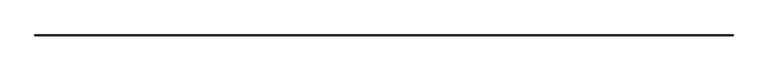
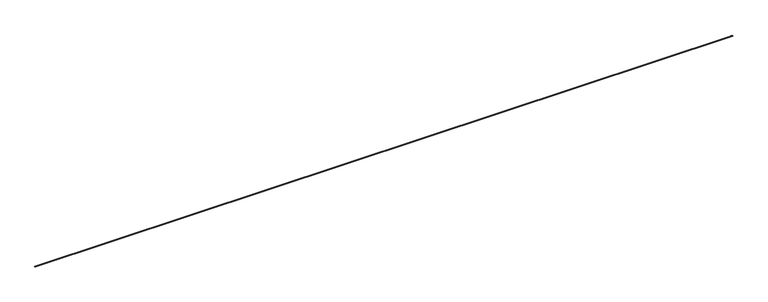
"""IFC4 building model written with IfcOpenShell, lengths in millimetres: proxy geometry, Generic Models 3:Generic Models 2:312240:Generic Models 2:312240 : Generic Models 3:Generic Models 2:312240:8 : Generic Models 3:Generic Models 2:312240:Generic Models 2:312240 : Generic Models 3:Generic Models 2:312240:300533."""

import ifcopenshell
import ifcopenshell.guid

model = None  # the IFC model being written
_history = None  # IfcOwnerHistory: only IFC2X3 demands one
_inside = {}  # id of a spatial element -> (the spatial element, [elements in it])
_under = {}  # id of a project, library or spatial element -> (it, [spatial elements below it])
_declared = {}  # id of a project -> (the project, [libraries it declares])
_typed = {}  # id of a type object -> (the type object, [elements of that type])
_made_of = {}  # id of a material, layer set ... -> (it, [elements and type objects made of it])


def new_model(schema):
    """Start an empty IFC model of exactly this schema.

    Asked for "IFC4X3", IfcOpenShell would pick the latest addendum, in which some entities
    have other attributes; the version numbers below select the first issue.
    IFC2X3 requires an IfcOwnerHistory on every rooted entity: one is made here for all.
    """
    global model, _history
    if schema == "IFC4X3":
        model = ifcopenshell.file(schema_version=(4, 3, 0, 0))
    else:
        model = ifcopenshell.file(schema=schema)
    _inside.clear()
    _under.clear()
    _declared.clear()
    _typed.clear()
    _made_of.clear()
    _history = None
    if model.schema == "IFC2X3":
        org = make("IfcOrganization", Name="unknown")
        user = make(
            "IfcPersonAndOrganization",
            ThePerson=make("IfcPerson", FamilyName="unknown"),
            TheOrganization=org,
        )
        app = make(
            "IfcApplication",
            ApplicationDeveloper=org,
            Version="unknown",
            ApplicationFullName="unknown",
            ApplicationIdentifier="unknown",
        )
        _history = make(
            "IfcOwnerHistory",
            OwningUser=user,
            OwningApplication=app,
            ChangeAction="ADDED",
            CreationDate=0,
        )
    return model


def make(cls, **values):
    """One entity of the class cls with the attributes given. An attribute that is None is left unset."""
    return model.create_entity(
        cls, **{name: value for name, value in values.items() if value is not None}
    )


def rooted(cls, **values):
    """An entity with a GlobalId (a new one), such as an element, a storey or a relation."""
    return make(cls, GlobalId=ifcopenshell.guid.new(), OwnerHistory=_history, **values)


def si_unit(unit_type, name, prefix=None):
    """IfcSIUnit, for example si_unit("LENGTHUNIT", "METRE", prefix="MILLI")."""
    return make("IfcSIUnit", UnitType=unit_type, Prefix=prefix, Name=name)


def assignment(units):
    """IfcUnitAssignment: the units of a project."""
    return None if units is None else make("IfcUnitAssignment", Units=units)


def point(xyz):
    """IfcCartesianPoint."""
    return None if xyz is None else make("IfcCartesianPoint", Coordinates=xyz)


def direction(xyz):
    """IfcDirection."""
    return None if xyz is None else make("IfcDirection", DirectionRatios=xyz)


def frame(location, z_axis=None, x_axis=None):
    """IfcAxis2Placement3D, a coordinate frame: its origin and axes. An axis left out is left unset."""
    return make(
        "IfcAxis2Placement3D",
        Location=point(location),
        Axis=direction(z_axis),
        RefDirection=direction(x_axis),
    )


def origin():
    """The frame at (0, 0, 0) with its axes left unset."""
    return frame((0.0, 0.0, 0.0))


def place(relative_to, where):
    """IfcLocalPlacement: puts the frame where relative to a parent placement (None: the world)."""
    return make(
        "IfcLocalPlacement", PlacementRelTo=relative_to, RelativePlacement=where
    )


def context(
    kind, dimensions, precision=None, world=None, true_north=None, identifier=None
):
    """IfcGeometricRepresentationContext, for example the 3D "Model" context."""
    return make(
        "IfcGeometricRepresentationContext",
        ContextIdentifier=identifier,
        ContextType=kind,
        CoordinateSpaceDimension=dimensions,
        Precision=precision,
        WorldCoordinateSystem=world,
        TrueNorth=true_north,
    )


def project(units=None, contexts=None):
    """IfcProject with its units and contexts."""
    return rooted(
        "IfcProject",
        Name="project",
        RepresentationContexts=contexts,
        UnitsInContext=assignment(units),
    )


def spatial(cls, under=None, at=None, **own):
    """A site, building, storey or space (cls), placed at a placement, below another one or the project."""
    s = rooted(cls, ObjectPlacement=at, **own)
    if under is not None:
        _under.setdefault(under.id(), (under, []))[1].append(s)
    return s


def polyline(points):
    """IfcPolyline through the points."""
    return make("IfcPolyline", Points=[point(p) for p in points])


def outline(outer, holes=None, kind="AREA"):
    """IfcArbitraryClosedProfileDef: a profile drawn as a closed curve; with holes, ...WithVoids."""
    if holes is None:
        return make("IfcArbitraryClosedProfileDef", ProfileType=kind, OuterCurve=outer)
    return make(
        "IfcArbitraryProfileDefWithVoids",
        ProfileType=kind,
        OuterCurve=outer,
        InnerCurves=holes,
    )


def extrude(swept, where, along, depth):
    """IfcExtrudedAreaSolid: the profile swept, set in the frame where, extruded along a direction by depth."""
    return make(
        "IfcExtrudedAreaSolid",
        SweptArea=swept,
        Position=where,
        ExtrudedDirection=direction(along),
        Depth=depth,
    )


def shape(context_of_items, identifier, shape_type, items):
    """IfcShapeRepresentation: the items that make up one representation, for example the "Body"."""
    return make(
        "IfcShapeRepresentation",
        ContextOfItems=context_of_items,
        RepresentationIdentifier=identifier,
        RepresentationType=shape_type,
        Items=items,
    )


def source(mapping_origin, context_of_items, identifier, shape_type, items):
    """IfcRepresentationMap: a shape defined once, which mapped items show again and again."""
    return make(
        "IfcRepresentationMap",
        MappingOrigin=mapping_origin,
        MappedRepresentation=shape(context_of_items, identifier, shape_type, items),
    )


def transform(
    local_origin,
    x_axis=None,
    y_axis=None,
    z_axis=None,
    scale=None,
    scale2=None,
    scale3=None,
    uniform=True,
):
    """IfcCartesianTransformationOperator3D, or its non-uniform kind. x_axis, y_axis, z_axis: its Axis1, 2, 3."""
    if uniform:
        return make(
            "IfcCartesianTransformationOperator3D",
            Axis1=direction(x_axis),
            Axis2=direction(y_axis),
            LocalOrigin=point(local_origin),
            Scale=scale,
            Axis3=direction(z_axis),
        )
    return make(
        "IfcCartesianTransformationOperator3DnonUniform",
        Axis1=direction(x_axis),
        Axis2=direction(y_axis),
        LocalOrigin=point(local_origin),
        Scale=scale,
        Axis3=direction(z_axis),
        Scale2=scale2,
        Scale3=scale3,
    )


def mapped(mapping_source, mapping_target):
    """IfcMappedItem: shows the shape of a source again, moved by a transform."""
    return make(
        "IfcMappedItem", MappingSource=mapping_source, MappingTarget=mapping_target
    )


def made_of(thing, what):
    """Note that an element or type object is made of a material, layer set ...; save() writes the relation."""
    if what is not None:
        _made_of.setdefault(what.id(), (what, []))[1].append(thing)
    return thing


def element(
    cls,
    number,
    at=None,
    inside=None,
    cuts=None,
    type_object=None,
    material=None,
    context=None,
    identifier="Body",
    shape_type=None,
    held_by="IfcProductDefinitionShape",
    body=None,
    shapes=None,
    **own,
):
    """One element of the class cls, such as IfcWall. Its Tag is "e" and its number.

    at: its placement. inside: the storey or other place that contains it. cuts: it is an
    opening in that element (IfcRelVoidsElement). A single representation is given by context,
    identifier, shape_type and body (its items); several are given by shapes. held_by: the class
    of the entity that holds the representations. save() writes the other relations.
    """
    e = rooted(cls, Tag="e%d" % number, ObjectPlacement=at, **own)
    if body is not None:
        shapes = [shape(context, identifier, shape_type, body)]
    if shapes is not None:
        e.Representation = make(held_by, Representations=shapes)
    if inside is not None:
        _inside.setdefault(inside.id(), (inside, []))[1].append(e)
    if cuts is not None:
        rooted(
            "IfcRelVoidsElement", RelatingBuildingElement=cuts, RelatedOpeningElement=e
        )
    if type_object is not None:
        _typed.setdefault(type_object.id(), (type_object, []))[1].append(e)
    return made_of(e, material)


def aggregate(whole, parts):
    """IfcRelAggregates: a whole, such as a stair, and the parts it consists of."""
    return rooted("IfcRelAggregates", RelatingObject=whole, RelatedObjects=parts)


def save(model, path):
    """Write the relations noted so far, then the file.

    IfcRelAggregates (storeys below a building ...), IfcRelContainedInSpatialStructure (elements
    in a storey), IfcRelDefinesByType, IfcRelAssociatesMaterial and IfcRelDeclares: one each for
    every whole, place, type object, material and project.
    """
    for whole, parts in _under.values():
        aggregate(whole, parts)
    for where, things in _inside.values():
        rooted(
            "IfcRelContainedInSpatialStructure",
            RelatedElements=things,
            RelatingStructure=where,
        )
    for kind, things in _typed.values():
        rooted("IfcRelDefinesByType", RelatedObjects=things, RelatingType=kind)
    for what, things in _made_of.values():
        rooted("IfcRelAssociatesMaterial", RelatedObjects=things, RelatingMaterial=what)
    for by, libraries in _declared.values():
        rooted("IfcRelDeclares", RelatingContext=by, RelatedDefinitions=libraries)
    model.write(path)


def generic_models_ac36fe79(model_context):
    return source(origin(), model_context, "Body", "SweptSolid", [
        extrude(outline(polyline([(-536697.1312083, -73.025), (-536697.1312083, -63.5), (-536696.3374583, -63.5), (-536696.3374583, -72.23125), (-536693.1624583, -72.23125), (-536693.1624583, -51.59375), (-536768.9802206, -51.59375), (-536768.9802206, 7.8475906), (-536768.1864706, 7.8475906), (-536768.1864706, -50.8), (-536692.3687083, -50.8), (-536692.3687083, -73.025), (-536697.1312083, -73.025)])), frame((593722.1429717, 0.0, 0.0), z_axis=(1.0, 0.0, 0.0), x_axis=(0.0, 1.0, 0.0)), (0.0, 0.0, 1.0), 50295.2437522),
    ])


if __name__ == "__main__":
    model = new_model("IFC4")
    model_context = context("Model", 3, world=origin())
    ifc_project = project(units=[si_unit("LENGTHUNIT", "METRE", prefix="MILLI")], contexts=[model_context])
    site = spatial("IfcSite", under=ifc_project)
    building = spatial("IfcBuilding", under=site)
    placement = place(None, origin())
    generic_models_shape = generic_models_ac36fe79(model_context)
    element("IfcBuildingElementProxy", 1, Name="Generic Models 3:Generic Models 2:312240:Generic Models 2:312240 : Generic Models 3:Generic Models 2:312240:8 : Generic Models 3:Generic Models 2:312240:Generic Models 2:312240 : Generic Models 3:Generic Models 2:312240:300533", ObjectType="Generic Models 3:Generic Models 2:312240:Generic Models 2:312240 : Generic Models 3:Generic Models 2:312240:8 : Generic Models 3:Generic Models 2:312240:Generic Models 2:312240 : Generic Models 3:Generic Models 2:312240:300533", at=placement, inside=building, context=model_context, shape_type="MappedRepresentation", body=[
        mapped(generic_models_shape, transform((0.0, 0.0, 0.0), x_axis=(1.0, 0.0, 0.0), y_axis=(0.0, 1.0, 0.0), z_axis=(0.0, 0.0, 1.0))),
    ])
    save(model, "model.ifc")

# Revit data of these elements
# Type "Generic Models 3:Generic Models 2:312240:Generic Models 2:312240 : Generic Models 3:Generic Models 2:312240:8 : Generic Models 3:Generic Models 2:312240:Generic Models 2:312240 : Generic Models 3:Generic Models 2:312240:300533"
#   NameOverride = "Generic Models 3:Generic Models 2:312240:Generic Models 2:312240 : Generic Models 3:Generic Models 2:312240:300533"
#   ObjectTypeOverride = "Generic Models 2:312240 : Generic Models 3:Generic Models 2:312240"
#   Reference = "Generic Models 2"
#   Tag = "300533"
# Element 1 (IfcBuildingElementProxy, "Generic Models 3:Generic Models 2:312240:Generic Models 2:312240 : Generic Models 3:Generic Models 2:312240:8 : Generic Models 3:Generic Models 2:312240:Generic Models 2:312240 : Generic Models 3:Generic Models 2:312240:300533")
#   Materials on its faces: "BRAKE METAL FLASHING WITH BACK & END DAMS"
# Materials
#   "BRAKE METAL FLASHING WITH BACK & END DAMS": class "Unassigned", colour RGB 182 182 182, transparency 0, Cost = 0
